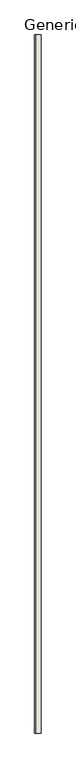
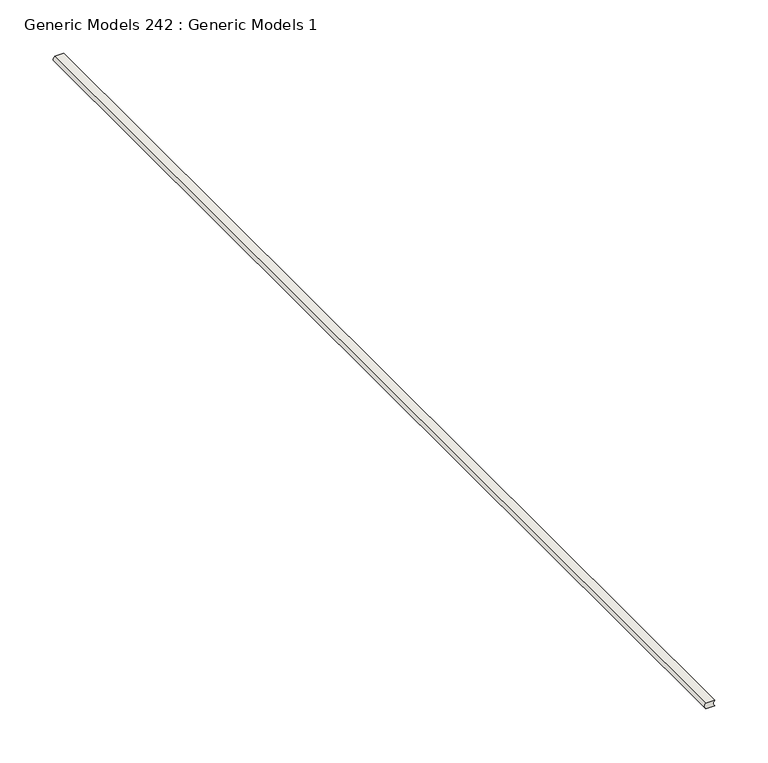
"""IFC4 building model written with IfcOpenShell, lengths in millimetres: wall geometry, Generic Models 242 : Generic Models 1."""

from ifc_helpers import new_model, si_unit, point, frame, frame_2d, origin, place, context, project, spatial, polyline, circle_curve, trimmed, segment, composite_curve, outline, extrude, source, transform, mapped, element, save


def generic_models_242_generic_models_1_1d67588c(model_context):
    return source(origin(), model_context, "Body", "SweptSolid", [
        extrude(outline(composite_curve([segment(trimmed(circle_curve(frame_2d((3051.175, 49802.7897405)), 4.3100275), [point((3048.0, 49799.875))], [point((3054.35, 49799.875))], True, "CARTESIAN"), True, "CONTINUOUS"), segment(polyline([(3054.35, 49799.875), (3054.35, 49790.35)]), True, "CONTINUOUS"), segment(trimmed(circle_curve(frame_2d((3051.175, 49793.2647405)), 4.3100275), [point((3054.35, 49790.35))], [point((3048.0, 49790.35))], False, "CARTESIAN"), True, "CONTINUOUS"), segment(polyline([(3048.0, 49790.35), (3048.0, 49799.875)]), True, "CONTINUOUS")], self_intersect=False)), frame((0.0, 0.0, 0.0), z_axis=(0.0, 1.0, 0.0), x_axis=(0.0, 0.0, 1.0)), (0.0, 0.0, 1.0), 1219.2),
    ])


if __name__ == "__main__":
    model = new_model("IFC4")
    model_context = context("Model", 3, world=origin())
    ifc_project = project(units=[si_unit("LENGTHUNIT", "METRE", prefix="MILLI")], contexts=[model_context])
    site = spatial("IfcSite", under=ifc_project)
    building = spatial("IfcBuilding", under=site)
    placement = place(None, origin())
    generic_models_242_generic_models_1_shape = generic_models_242_generic_models_1_1d67588c(model_context)
    element("IfcWall", 1, ObjectType="Generic Models 242 : Generic Models 1", at=placement, inside=building, context=model_context, shape_type="MappedRepresentation", body=[
        mapped(generic_models_242_generic_models_1_shape, transform((0.0, 0.0, 0.0), x_axis=(1.0, 0.0, 0.0), y_axis=(0.0, 1.0, 0.0), z_axis=(0.0, 0.0, 1.0))),
    ])
    save(model, "model.ifc")

# Revit data of these elements
# Element 1 (IfcWall, "Generic Models 242 : Generic Models 1")
#   Materials on its faces: "ACOUSTICAL SEALANT"
# Materials
#   "ACOUSTICAL SEALANT": class "Unassigned", colour RGB 120 120 120, transparency 0, Cost = 0
